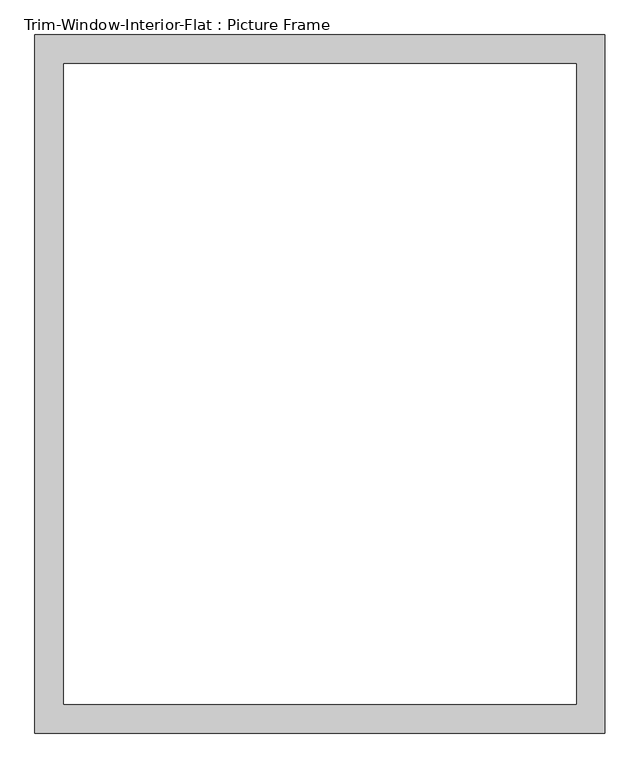
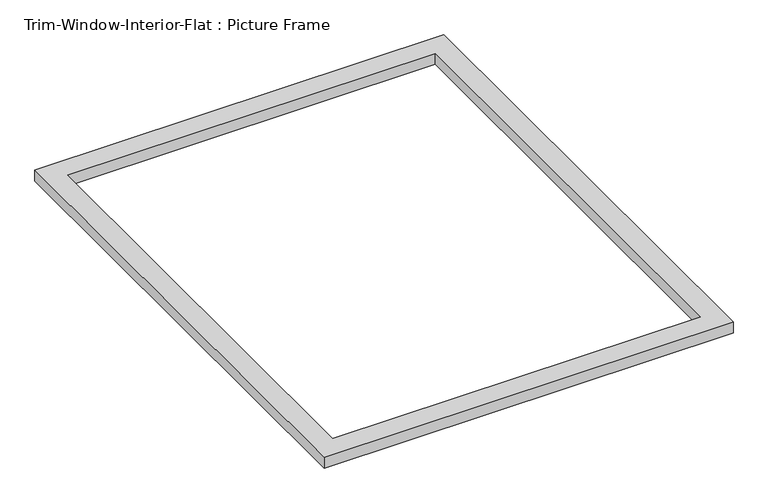
"""IFC4 building model written with IfcOpenShell, lengths in millimetres: proxy geometry, Trim-Window-Interior-Flat : Picture Frame."""

from ifc_helpers import new_model, si_unit, origin, origin_with_axes, place, context, project, spatial, polyline, outline, extrude, source, transform, mapped, element, save


def trim_window_interior_flat_picture_frame_b488ca0e(model_context):
    return source(origin(), model_context, "Body", "SweptSolid", [
        extrude(outline(polyline([(565.15, 44.45), (565.15, -1339.85), (-565.15, -1339.85), (-565.15, 44.45), (565.15, 44.45)]), holes=[polyline([(508.0, -12.7), (-508.0, -12.7), (-508.0, -1282.7), (508.0, -1282.7), (508.0, -12.7)])]), origin_with_axes(), (0.0, 0.0, 1.0), 31.75),
    ])


if __name__ == "__main__":
    model = new_model("IFC4")
    model_context = context("Model", 3, world=origin())
    ifc_project = project(units=[si_unit("LENGTHUNIT", "METRE", prefix="MILLI")], contexts=[model_context])
    site = spatial("IfcSite", under=ifc_project)
    building = spatial("IfcBuilding", under=site)
    placement = place(None, origin())
    trim_window_interior_flat_picture_frame_shape = trim_window_interior_flat_picture_frame_b488ca0e(model_context)
    element("IfcBuildingElementProxy", 1, Name="Trim-Window-Interior-Flat : Picture Frame", ObjectType="Trim-Window-Interior-Flat : Picture Frame", at=placement, inside=building, context=model_context, shape_type="MappedRepresentation", body=[
        mapped(trim_window_interior_flat_picture_frame_shape, transform((0.0, 0.0, 0.0), x_axis=(1.0, 0.0, 0.0), y_axis=(0.0, 1.0, 0.0), z_axis=(0.0, 0.0, 1.0))),
    ])
    save(model, "model.ifc")

# Revit data of these elements
# Type "Trim-Window-Interior-Flat : Picture Frame"
#   Trim Thickness_Picture Frame = 0' - 1 1/4"
#   Trim Width = 0' - 2 1/4"
#   Trim Thickness_with Sill = 0' - 0 3/4"
#   Sill Thickness = 0' - 1 1/4"
#   Opening Width [instance default] = 2' - 0"
#   Opening Height [instance default] = 3' - 0"
#   Default Elevation = 4' - 0"
#   Sill = no
#   Picture Frame = yes
#   Trim Material [instance default] = none
# Element 1 (IfcBuildingElementProxy, "Trim-Window-Interior-Flat : Picture Frame")
#   Opening Width = 3' - 5"
#   Opening Height = 4' - 3"
#   Trim Material = 1X WOOD COMPOSITE TRIM
#   Materials on its faces: "1X WOOD COMPOSITE TRIM"
# Materials
#   "1X WOOD COMPOSITE TRIM": class "Generic", colour RGB 88 61 61, transparency 0, Cost = 0
